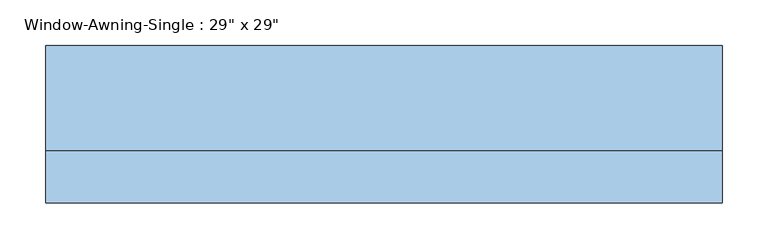
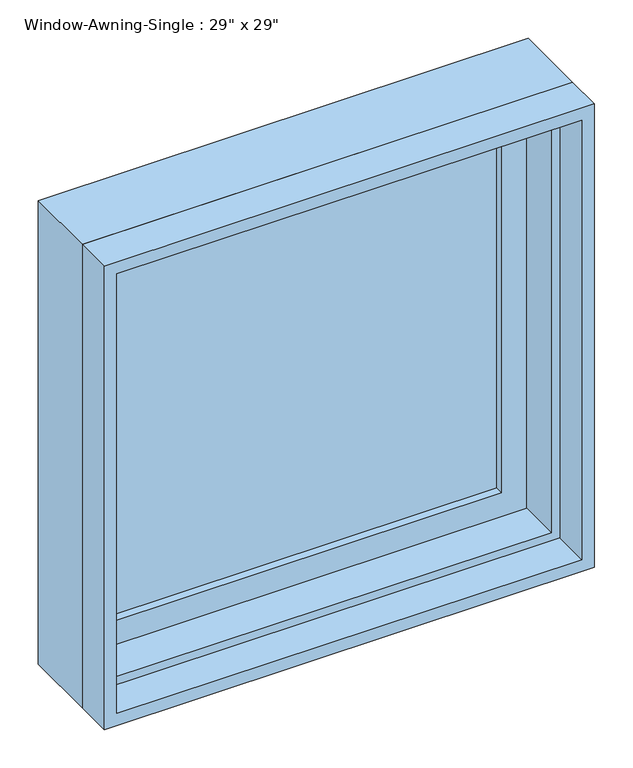
"""IFC4 building model written with IfcOpenShell, lengths in millimetres: window geometry."""

from ifc_helpers import new_model, si_unit, frame, origin, place, context, project, spatial, polyline, outline, extrude, faceted_brep, source, transform, mapped, element, save


def window_d74d2e6b(model_context):
    return source(origin(), model_context, "Body", "SolidModel", [
        faceted_brep([(355.6, 44.45, 927.1), (355.6, 95.25, 927.1), (-355.6, 95.25, 927.1), (-355.6, 44.45, 927.1), (336.55, -19.05, 946.15), (336.55, 44.45, 946.15), (-336.55, 44.45, 946.15), (-336.55, -19.05, 946.15), (368.3, 95.25, 914.4), (368.3, -19.05, 914.4), (-368.3, -19.05, 914.4), (-368.3, 95.25, 914.4), (-355.6, 95.25, 1638.3), (-355.6, 44.45, 1638.3), (-336.55, 44.45, 1619.25), (-336.55, -19.05, 1619.25), (-368.3, -19.05, 1651.0), (-368.3, 95.25, 1651.0), (355.6, 95.25, 1638.3), (355.6, 44.45, 1638.3), (336.55, 44.45, 1619.25), (336.55, -19.05, 1619.25), (368.3, -19.05, 1651.0), (368.3, 95.25, 1651.0)], [[[0, 1, 2, 3]], [[4, 5, 6, 7]], [[8, 9, 10, 11]], [[3, 2, 12, 13]], [[7, 6, 14, 15]], [[11, 10, 16, 17]], [[13, 12, 18, 19]], [[15, 14, 20, 21]], [[17, 16, 22, 23]], [[11, 17, 23, 8], [1, 18, 12, 2]], [[19, 18, 1, 0]], [[3, 13, 19, 0], [5, 20, 14, 6]], [[21, 20, 5, 4]], [[9, 22, 16, 10], [7, 15, 21, 4]], [[23, 22, 9, 8]]]),
        extrude(outline(polyline([(298.45, 76.2), (298.45, 69.85), (-298.45, 69.85), (-298.45, 76.2), (298.45, 76.2)])), frame((0.0, 0.0, 984.25), z_axis=(0.0, 0.0, 1.0), x_axis=(1.0, 0.0, 0.0)), (0.0, 0.0, 1.0), 596.9),
        extrude(outline(polyline([(298.45, 63.5), (298.45, 57.15), (-298.45, 57.15), (-298.45, 63.5), (298.45, 63.5)])), frame((0.0, 0.0, 984.25), z_axis=(0.0, 0.0, 1.0), x_axis=(1.0, 0.0, 0.0)), (0.0, 0.0, 1.0), 596.9),
        extrude(outline(polyline([(927.1, -355.6), (927.1, 355.6), (1638.3, 355.6), (1638.3, -355.6), (927.1, -355.6)]), holes=[polyline([(1581.15, -298.45), (1581.15, 298.45), (984.25, 298.45), (984.25, -298.45), (1581.15, -298.45)])]), frame((0.0, 44.45, 0.0), z_axis=(0.0, 1.0, 0.0), x_axis=(0.0, 0.0, 1.0)), (0.0, 0.0, 1.0), 44.45),
        extrude(outline(polyline([(1651.0, -368.3), (914.4, -368.3), (914.4, 368.3), (1651.0, 368.3), (1651.0, -368.3)]), holes=[polyline([(1631.95, -349.25), (1631.95, 349.25), (933.45, 349.25), (933.45, -349.25), (1631.95, -349.25)])]), frame((0.0, -76.2, 0.0), z_axis=(0.0, 1.0, 0.0), x_axis=(0.0, 0.0, 1.0)), (0.0, 0.0, 1.0), 57.15),
    ])


if __name__ == "__main__":
    model = new_model("IFC4")
    model_context = context("Model", 3, world=origin())
    ifc_project = project(units=[si_unit("LENGTHUNIT", "METRE", prefix="MILLI")], contexts=[model_context])
    site = spatial("IfcSite", under=ifc_project)
    building = spatial("IfcBuilding", under=site)
    placement = place(None, origin())
    window_shape = window_d74d2e6b(model_context)
    element("IfcWindow", 1, ObjectType="Window-Awning-Single : 29\" x 29\"", at=placement, inside=building, context=model_context, shape_type="MappedRepresentation", body=[
        mapped(window_shape, transform((0.0, 0.0, 0.0), x_axis=(1.0, 0.0, 0.0), y_axis=(0.0, 1.0, 0.0), z_axis=(0.0, 0.0, 1.0))),
    ])
    save(model, "model.ifc")

# Revit data of these elements
# Type "Window-Awning-Single : 29\" x 29\""
#   Type Mark = "13"
#   Fire Rating = "0.5h"
#   Assembly Code = "B2020100"
#   Analytic Construction = "Double glazing - domestic"
#   Window Inset [instance default] = 0' - 0"
#   Wall Thickness [instance default] = 0' - 6"
#   Visual Light Transmittance = 0.81
#   Thermal Resistance (R) = 0.319569 (m²·K)/W
#   Solar Heat Gain Coefficient = 0.76
#   Rough Width = 2' - 5 1/2"
#   Rough Height = 2' - 5 1/2"
#   Interior Wall Closure [instance default] = 0' - 2 1/4"
#   Height = 2' - 5"
#   Heat Transfer Coefficient (U) = 3.12929 W/(m²·K)
#   Frame Extension [instance default] = 0' - 0 1/4"
#   Exterior Wall Closure [instance default] = 0' - 1 1/4"
#   Extension Jamb [instance default] = 0' - 2 1/4"
#   Default Sill Height = 3' - 0"
#   Width = 2' - 5"
#   Muntin Visibility = yes
#   Interior Trim Visibility [instance default] = yes
#   Exterior Trim Visibility [instance default] = yes
#   Extension Jamb Visibility [instance default] = yes
#   Muntin Pattern = Muntin Pattern_2x2 : Muntin Pattern_2x2
#   Interior Trim Material = Wood - Stained
#   Interior Trim = Trim-Window-Interior-Flat : Picture Frame
#   Interior Frame Material = Wood - Stained
#   Glass Panel Material = Glass
#   Exterior Trim Material = Clad - White
#   Exterior Trim = Trim-Window-Exterior-Flat : with Sill
#   Exterior Frame Material = Clad - White
#   Wall Closure = (empty or 0)
# Element 1 (IfcWindow, "Window-Awning-Single : 29\" x 29\"")
#   Materials on its faces: "Wood - Stained", "Glass", "Clad - White"
# Materials
#   "Wood - Stained": class "Wood", colour RGB 224 178 126, transparency 0, Cost = 0
#   "Glass": class "Glass", colour RGB 236 240 239, transparency 0.85, Description = "Soda Lime Glass", Cost = 0
#   "Clad - White": class "Wood", colour RGB 242 242 238, transparency 0, Cost = 0
